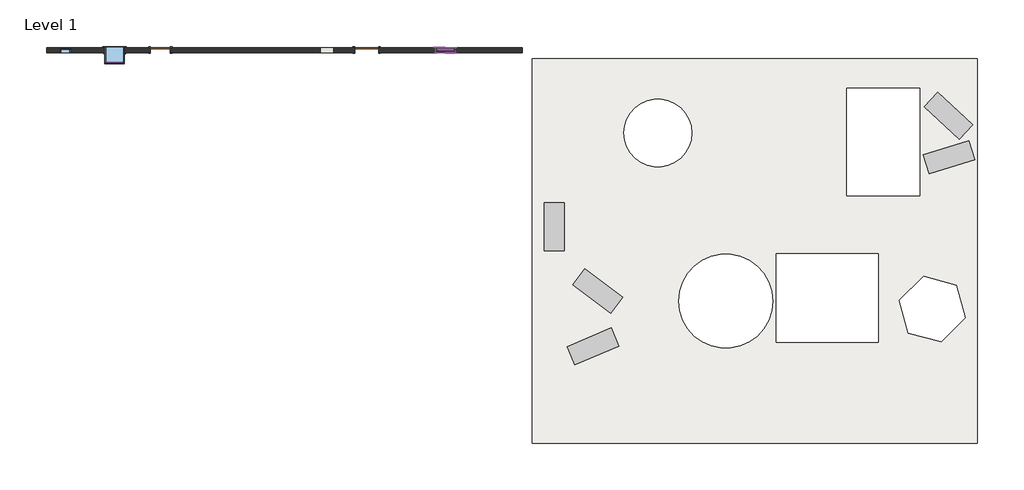
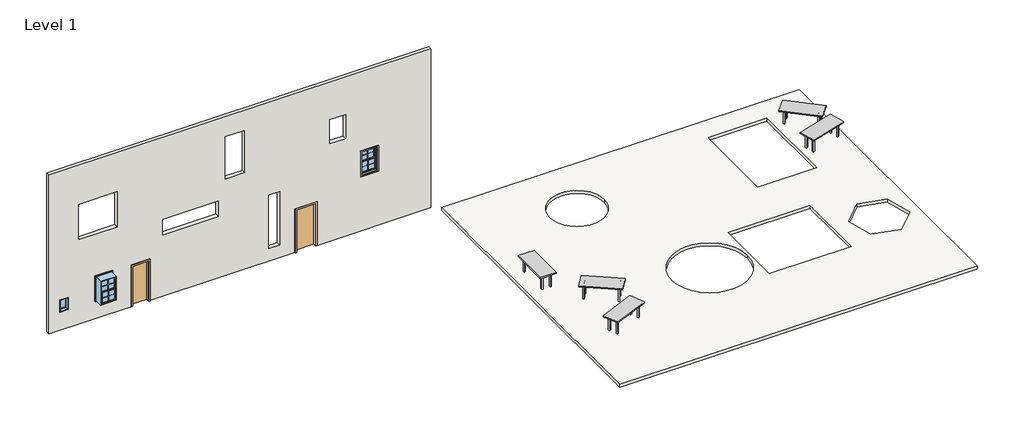
# One storey: 8 proxies, 5 furniture elements, 3 windows, 2 doors, 1 slab, 1 wall.
"""IFC4 building model written with IfcOpenShell, lengths in millimetres."""

import ifcopenshell
import ifcopenshell.guid

model = None  # the IFC model being written
_history = None  # IfcOwnerHistory: only IFC2X3 demands one
_inside = {}  # id of a spatial element -> (the spatial element, [elements in it])
_under = {}  # id of a project, library or spatial element -> (it, [spatial elements below it])
_declared = {}  # id of a project -> (the project, [libraries it declares])
_typed = {}  # id of a type object -> (the type object, [elements of that type])
_made_of = {}  # id of a material, layer set ... -> (it, [elements and type objects made of it])


def new_model(schema):
    """Start an empty IFC model of exactly this schema.

    Asked for "IFC4X3", IfcOpenShell would pick the latest addendum, in which some entities
    have other attributes; the version numbers below select the first issue.
    IFC2X3 requires an IfcOwnerHistory on every rooted entity: one is made here for all.
    """
    global model, _history
    if schema == "IFC4X3":
        model = ifcopenshell.file(schema_version=(4, 3, 0, 0))
    else:
        model = ifcopenshell.file(schema=schema)
    _inside.clear()
    _under.clear()
    _declared.clear()
    _typed.clear()
    _made_of.clear()
    _history = None
    if model.schema == "IFC2X3":
        org = make("IfcOrganization", Name="unknown")
        user = make(
            "IfcPersonAndOrganization",
            ThePerson=make("IfcPerson", FamilyName="unknown"),
            TheOrganization=org,
        )
        app = make(
            "IfcApplication",
            ApplicationDeveloper=org,
            Version="unknown",
            ApplicationFullName="unknown",
            ApplicationIdentifier="unknown",
        )
        _history = make(
            "IfcOwnerHistory",
            OwningUser=user,
            OwningApplication=app,
            ChangeAction="ADDED",
            CreationDate=0,
        )
    return model


def make(cls, **values):
    """One entity of the class cls with the attributes given. An attribute that is None is left unset."""
    return model.create_entity(
        cls, **{name: value for name, value in values.items() if value is not None}
    )


def rooted(cls, **values):
    """An entity with a GlobalId (a new one), such as an element, a storey or a relation."""
    return make(cls, GlobalId=ifcopenshell.guid.new(), OwnerHistory=_history, **values)


def si_unit(unit_type, name, prefix=None):
    """IfcSIUnit, for example si_unit("LENGTHUNIT", "METRE", prefix="MILLI")."""
    return make("IfcSIUnit", UnitType=unit_type, Prefix=prefix, Name=name)


def assignment(units):
    """IfcUnitAssignment: the units of a project."""
    return None if units is None else make("IfcUnitAssignment", Units=units)


def point(xyz):
    """IfcCartesianPoint."""
    return None if xyz is None else make("IfcCartesianPoint", Coordinates=xyz)


def direction(xyz):
    """IfcDirection."""
    return None if xyz is None else make("IfcDirection", DirectionRatios=xyz)


def frame(location, z_axis=None, x_axis=None):
    """IfcAxis2Placement3D, a coordinate frame: its origin and axes. An axis left out is left unset."""
    return make(
        "IfcAxis2Placement3D",
        Location=point(location),
        Axis=direction(z_axis),
        RefDirection=direction(x_axis),
    )


def frame_2d(location, x_axis=None):
    """IfcAxis2Placement2D, a coordinate frame in the plane: its origin and x axis."""
    return make(
        "IfcAxis2Placement2D", Location=point(location), RefDirection=direction(x_axis)
    )


def origin():
    """The frame at (0, 0, 0) with its axes left unset."""
    return frame((0.0, 0.0, 0.0))


def origin_with_axes():
    """The frame at (0, 0, 0) with the z axis (0, 0, 1) and the x axis (1, 0, 0) written out."""
    return frame((0.0, 0.0, 0.0), z_axis=(0.0, 0.0, 1.0), x_axis=(1.0, 0.0, 0.0))


def place(relative_to, where):
    """IfcLocalPlacement: puts the frame where relative to a parent placement (None: the world)."""
    return make(
        "IfcLocalPlacement", PlacementRelTo=relative_to, RelativePlacement=where
    )


def context(
    kind, dimensions, precision=None, world=None, true_north=None, identifier=None
):
    """IfcGeometricRepresentationContext, for example the 3D "Model" context."""
    return make(
        "IfcGeometricRepresentationContext",
        ContextIdentifier=identifier,
        ContextType=kind,
        CoordinateSpaceDimension=dimensions,
        Precision=precision,
        WorldCoordinateSystem=world,
        TrueNorth=true_north,
    )


def project(units=None, contexts=None):
    """IfcProject with its units and contexts."""
    return rooted(
        "IfcProject",
        Name="project",
        RepresentationContexts=contexts,
        UnitsInContext=assignment(units),
    )


def spatial(cls, under=None, at=None, **own):
    """A site, building, storey or space (cls), placed at a placement, below another one or the project."""
    s = rooted(cls, ObjectPlacement=at, **own)
    if under is not None:
        _under.setdefault(under.id(), (under, []))[1].append(s)
    return s


def polyline(points):
    """IfcPolyline through the points."""
    return make("IfcPolyline", Points=[point(p) for p in points])


def circle_curve(where, radius):
    """IfcCircle in the frame where."""
    return make("IfcCircle", Position=where, Radius=radius)


def trimmed(basis, trim1, trim2, sense, master):
    """IfcTrimmedCurve: the piece of a basis curve between two trims."""
    return make(
        "IfcTrimmedCurve",
        BasisCurve=basis,
        Trim1=trim1,
        Trim2=trim2,
        SenseAgreement=sense,
        MasterRepresentation=master,
    )


def segment(curve, same_sense, transition):
    """IfcCompositeCurveSegment."""
    return make(
        "IfcCompositeCurveSegment",
        Transition=transition,
        SameSense=same_sense,
        ParentCurve=curve,
    )


def composite_curve(segments, self_intersect=None):
    """IfcCompositeCurve: segments joined end to end."""
    return make("IfcCompositeCurve", Segments=segments, SelfIntersect=self_intersect)


def outline(outer, holes=None, kind="AREA"):
    """IfcArbitraryClosedProfileDef: a profile drawn as a closed curve; with holes, ...WithVoids."""
    if holes is None:
        return make("IfcArbitraryClosedProfileDef", ProfileType=kind, OuterCurve=outer)
    return make(
        "IfcArbitraryProfileDefWithVoids",
        ProfileType=kind,
        OuterCurve=outer,
        InnerCurves=holes,
    )


def extrude(swept, where, along, depth):
    """IfcExtrudedAreaSolid: the profile swept, set in the frame where, extruded along a direction by depth."""
    return make(
        "IfcExtrudedAreaSolid",
        SweptArea=swept,
        Position=where,
        ExtrudedDirection=direction(along),
        Depth=depth,
    )


def shape(context_of_items, identifier, shape_type, items):
    """IfcShapeRepresentation: the items that make up one representation, for example the "Body"."""
    return make(
        "IfcShapeRepresentation",
        ContextOfItems=context_of_items,
        RepresentationIdentifier=identifier,
        RepresentationType=shape_type,
        Items=items,
    )


def source(mapping_origin, context_of_items, identifier, shape_type, items):
    """IfcRepresentationMap: a shape defined once, which mapped items show again and again."""
    return make(
        "IfcRepresentationMap",
        MappingOrigin=mapping_origin,
        MappedRepresentation=shape(context_of_items, identifier, shape_type, items),
    )


def transform(
    local_origin,
    x_axis=None,
    y_axis=None,
    z_axis=None,
    scale=None,
    scale2=None,
    scale3=None,
    uniform=True,
):
    """IfcCartesianTransformationOperator3D, or its non-uniform kind. x_axis, y_axis, z_axis: its Axis1, 2, 3."""
    if uniform:
        return make(
            "IfcCartesianTransformationOperator3D",
            Axis1=direction(x_axis),
            Axis2=direction(y_axis),
            LocalOrigin=point(local_origin),
            Scale=scale,
            Axis3=direction(z_axis),
        )
    return make(
        "IfcCartesianTransformationOperator3DnonUniform",
        Axis1=direction(x_axis),
        Axis2=direction(y_axis),
        LocalOrigin=point(local_origin),
        Scale=scale,
        Axis3=direction(z_axis),
        Scale2=scale2,
        Scale3=scale3,
    )


def mapped(mapping_source, mapping_target):
    """IfcMappedItem: shows the shape of a source again, moved by a transform."""
    return make(
        "IfcMappedItem", MappingSource=mapping_source, MappingTarget=mapping_target
    )


def made_of(thing, what):
    """Note that an element or type object is made of a material, layer set ...; save() writes the relation."""
    if what is not None:
        _made_of.setdefault(what.id(), (what, []))[1].append(thing)
    return thing


def element(
    cls,
    number,
    at=None,
    inside=None,
    cuts=None,
    type_object=None,
    material=None,
    context=None,
    identifier="Body",
    shape_type=None,
    held_by="IfcProductDefinitionShape",
    body=None,
    shapes=None,
    **own,
):
    """One element of the class cls, such as IfcWall. Its Tag is "e" and its number.

    at: its placement. inside: the storey or other place that contains it. cuts: it is an
    opening in that element (IfcRelVoidsElement). A single representation is given by context,
    identifier, shape_type and body (its items); several are given by shapes. held_by: the class
    of the entity that holds the representations. save() writes the other relations.
    """
    e = rooted(cls, Tag="e%d" % number, ObjectPlacement=at, **own)
    if body is not None:
        shapes = [shape(context, identifier, shape_type, body)]
    if shapes is not None:
        e.Representation = make(held_by, Representations=shapes)
    if inside is not None:
        _inside.setdefault(inside.id(), (inside, []))[1].append(e)
    if cuts is not None:
        rooted(
            "IfcRelVoidsElement", RelatingBuildingElement=cuts, RelatedOpeningElement=e
        )
    if type_object is not None:
        _typed.setdefault(type_object.id(), (type_object, []))[1].append(e)
    return made_of(e, material)


def aggregate(whole, parts):
    """IfcRelAggregates: a whole, such as a stair, and the parts it consists of."""
    return rooted("IfcRelAggregates", RelatingObject=whole, RelatedObjects=parts)


def save(model, path):
    """Write the relations noted so far, then the file.

    IfcRelAggregates (storeys below a building ...), IfcRelContainedInSpatialStructure (elements
    in a storey), IfcRelDefinesByType, IfcRelAssociatesMaterial and IfcRelDeclares: one each for
    every whole, place, type object, material and project.
    """
    for whole, parts in _under.values():
        aggregate(whole, parts)
    for where, things in _inside.values():
        rooted(
            "IfcRelContainedInSpatialStructure",
            RelatedElements=things,
            RelatingStructure=where,
        )
    for kind, things in _typed.values():
        rooted("IfcRelDefinesByType", RelatedObjects=things, RelatingType=kind)
    for what, things in _made_of.values():
        rooted("IfcRelAssociatesMaterial", RelatedObjects=things, RelatingMaterial=what)
    for by, libraries in _declared.values():
        rooted("IfcRelDeclares", RelatingContext=by, RelatedDefinitions=libraries)
    model.write(path)


def m_muntin_pattern_2x2_m_muntin_pattern_2x2_aaec3afb(model_context):
    return source(origin(), model_context, "Body", "SweptSolid", [
        extrude(outline(polyline([(257.1375, -6.35), (257.1375, -298.8), (244.4375, -298.8), (244.4375, -6.35), (0.0, -6.35), (0.0, 6.35), (244.4375, 6.35), (244.4375, 298.8), (257.1375, 298.8), (257.1375, 6.35), (501.575, 6.35), (501.575, -6.35), (257.1375, -6.35)])), frame((0.0, 9.525, 0.0), z_axis=(0.0, 1.0, 0.0), x_axis=(0.0, 0.0, 1.0)), (0.0, 0.0, 1.0), 12.7),
        extrude(outline(polyline([(257.1375, -6.35), (257.1375, -298.8), (244.4375, -298.8), (244.4375, -6.35), (0.0, -6.35), (0.0, 6.35), (244.4375, 6.35), (244.4375, 298.8), (257.1375, 298.8), (257.1375, 6.35), (501.575, 6.35), (501.575, -6.35), (257.1375, -6.35)])), frame((0.0, -22.225, 0.0), z_axis=(0.0, 1.0, 0.0), x_axis=(0.0, 0.0, 1.0)), (0.0, 0.0, 1.0), 12.7),
    ])


def m_trim_window_exterior_flat_with_sill_e7ff6350(model_context):
    return source(origin(), model_context, "Body", "SweptSolid", [
        extrude(outline(polyline([(435.0, -1220.4323709), (435.0, -1280.4323709), (-435.0, -1280.4323709), (-435.0, -1220.4323709), (435.0, -1220.4323709)])), origin_with_axes(), (0.0, 0.0, 1.0), 19.05),
        extrude(outline(polyline([(-1230.0, 38.1), (-1202.4580645, 38.1), (-1200.0, 19.05), (-1200.0, 0.0), (-1220.4323709, 0.0), (-1220.4323709, 19.05), (-1230.0, 19.05), (-1230.0, 38.1)])), frame((-447.7, 0.0, 0.0), z_axis=(1.0, 0.0, 0.0), x_axis=(0.0, 1.0, 0.0)), (0.0, 0.0, 1.0), 895.4),
        extrude(outline(polyline([(-435.0, 60.0), (435.0, 60.0), (435.0, -1200.0), (375.0, -1200.0), (375.0, 0.0), (-375.0, 0.0), (-375.0, -1200.0), (-435.0, -1200.0), (-435.0, 60.0)])), origin_with_axes(), (0.0, 0.0, 1.0), 19.05),
    ])


def m_trim_window_interior_flat_picture_frame_31bd2320(model_context):
    return source(origin(), model_context, "Body", "SweptSolid", [
        extrude(outline(polyline([(422.3, 47.3), (422.3, -1247.3), (-422.3, -1247.3), (-422.3, 47.3), (422.3, 47.3)]), holes=[polyline([(362.3, -12.7), (-362.3, -12.7), (-362.3, -1187.3), (362.3, -1187.3), (362.3, -12.7)])]), origin_with_axes(), (0.0, 0.0, 1.0), 30.0),
    ])


def m_single_flush_0762_x_2032mm_0c256fab(model_context):
    return source(origin(), model_context, "Body", "SweptSolid", [
        extrude(outline(polyline([(2108.0, -457.0), (0.0, -457.0), (0.0, -381.0), (2032.0, -381.0), (2032.0, 381.0), (0.0, 381.0), (0.0, 457.0), (2108.0, 457.0), (2108.0, -457.0)])), frame((0.0, 100.0, 0.0), z_axis=(0.0, 1.0, 0.0), x_axis=(0.0, 0.0, 1.0)), (0.0, 0.0, 1.0), 25.0),
        extrude(outline(polyline([(2108.0, 457.0), (2108.0, -457.0), (0.0, -457.0), (0.0, -381.0), (2032.0, -381.0), (2032.0, 381.0), (0.0, 381.0), (0.0, 457.0), (2108.0, 457.0)])), frame((0.0, -125.0, 0.0), z_axis=(0.0, 1.0, 0.0), x_axis=(0.0, 0.0, 1.0)), (0.0, 0.0, 1.0), 25.0),
        extrude(outline(polyline([(381.0, 49.0), (-381.0, 49.0), (-381.0, 100.0), (381.0, 100.0), (381.0, 49.0)])), origin_with_axes(), (0.0, 0.0, 1.0), 2032.0),
    ])


def m_single_flush_0915_x_2134mm_727434cd(model_context):
    return source(origin(), model_context, "Body", "SweptSolid", [
        extrude(outline(polyline([(2210.0, -533.5), (0.0, -533.5), (0.0, -457.5), (2134.0, -457.5), (2134.0, 457.5), (0.0, 457.5), (0.0, 533.5), (2210.0, 533.5), (2210.0, -533.5)])), frame((0.0, -125.0, 0.0), z_axis=(0.0, 1.0, 0.0), x_axis=(0.0, 0.0, 1.0)), (0.0, 0.0, 1.0), 25.0),
        extrude(outline(polyline([(2210.0, 533.5), (2210.0, -533.5), (0.0, -533.5), (0.0, -457.5), (2134.0, -457.5), (2134.0, 457.5), (0.0, 457.5), (0.0, 533.5), (2210.0, 533.5)])), frame((0.0, 100.0, 0.0), z_axis=(0.0, 1.0, 0.0), x_axis=(0.0, 0.0, 1.0)), (0.0, 0.0, 1.0), 25.0),
        extrude(outline(polyline([(457.5, -49.0), (457.5, -100.0), (-457.5, -100.0), (-457.5, -49.0), (457.5, -49.0)])), origin_with_axes(), (0.0, 0.0, 1.0), 2134.0),
    ])


def m_table_rectangular_1830_x_0762mm_a0b3b7a0(model_context):
    return source(origin(), model_context, "Body", "SweptSolid", [
        extrude(outline(polyline([(699.1, 190.5), (699.1, 165.1), (-699.1, 165.1), (-699.1, 190.5), (699.1, 190.5)])), frame((0.0, 0.0, 609.6), z_axis=(0.0, 0.0, 1.0), x_axis=(1.0, 0.0, 0.0)), (0.0, 0.0, 1.0), 101.6),
        extrude(outline(polyline([(699.1, -190.5), (-699.1, -190.5), (-699.1, -165.1), (699.1, -165.1), (699.1, -190.5)])), frame((0.0, 0.0, 609.6), z_axis=(0.0, 0.0, 1.0), x_axis=(1.0, 0.0, 0.0)), (0.0, 0.0, 1.0), 101.6),
        extrude(outline(polyline([(-711.8, -165.1), (-737.2, -165.1), (-737.2, 165.1), (-711.8, 165.1), (-711.8, -165.1)])), frame((0.0, 0.0, 609.6), z_axis=(0.0, 0.0, 1.0), x_axis=(1.0, 0.0, 0.0)), (0.0, 0.0, 1.0), 101.6),
        extrude(outline(polyline([(711.8, -165.1), (711.8, 165.1), (737.2, 165.1), (737.2, -165.1), (711.8, -165.1)])), frame((0.0, 0.0, 609.6), z_axis=(0.0, 0.0, 1.0), x_axis=(1.0, 0.0, 0.0)), (0.0, 0.0, 1.0), 101.6),
        extrude(outline(polyline([(915.0, 381.0), (915.0, -381.0), (-915.0, -381.0), (-915.0, 381.0), (915.0, 381.0)])), frame((0.0, 0.0, 711.2), z_axis=(0.0, 0.0, 1.0), x_axis=(1.0, 0.0, 0.0)), (0.0, 0.0, 1.0), 50.8),
        extrude(outline(polyline([(-699.1, 228.6), (-699.1, 165.1), (-762.6, 165.1), (-762.6, 228.6), (-699.1, 228.6)])), origin_with_axes(), (0.0, 0.0, 1.0), 711.2),
        extrude(outline(polyline([(699.1, 228.6), (762.6, 228.6), (762.6, 165.1), (699.1, 165.1), (699.1, 228.6)])), origin_with_axes(), (0.0, 0.0, 1.0), 711.2),
        extrude(outline(polyline([(-699.1, -228.6), (-762.6, -228.6), (-762.6, -165.1), (-699.1, -165.1), (-699.1, -228.6)])), origin_with_axes(), (0.0, 0.0, 1.0), 711.2),
        extrude(outline(polyline([(699.1, -228.6), (699.1, -165.1), (762.6, -165.1), (762.6, -228.6), (699.1, -228.6)])), origin_with_axes(), (0.0, 0.0, 1.0), 711.2),
    ])


def m_table_rectangular_1830_x_0762mm_ec068ed4(model_context):
    return source(origin(), model_context, "Body", "SweptSolid", [
        extrude(outline(polyline([(699.1, -190.5), (-699.1, -190.5), (-699.1, -165.1), (699.1, -165.1), (699.1, -190.5)])), frame((0.0, 0.0, 609.6), z_axis=(0.0, 0.0, 1.0), x_axis=(1.0, 0.0, 0.0)), (0.0, 0.0, 1.0), 101.6),
        extrude(outline(polyline([(699.1, 190.5), (699.1, 165.1), (-699.1, 165.1), (-699.1, 190.5), (699.1, 190.5)])), frame((0.0, 0.0, 609.6), z_axis=(0.0, 0.0, 1.0), x_axis=(1.0, 0.0, 0.0)), (0.0, 0.0, 1.0), 101.6),
        extrude(outline(polyline([(-711.8, 165.1), (-711.8, -165.1), (-737.2, -165.1), (-737.2, 165.1), (-711.8, 165.1)])), frame((0.0, 0.0, 609.6), z_axis=(0.0, 0.0, 1.0), x_axis=(1.0, 0.0, 0.0)), (0.0, 0.0, 1.0), 101.6),
        extrude(outline(polyline([(711.8, 165.1), (737.2, 165.1), (737.2, -165.1), (711.8, -165.1), (711.8, 165.1)])), frame((0.0, 0.0, 609.6), z_axis=(0.0, 0.0, 1.0), x_axis=(1.0, 0.0, 0.0)), (0.0, 0.0, 1.0), 101.6),
        extrude(outline(polyline([(915.0, -381.0), (-915.0, -381.0), (-915.0, 381.0), (915.0, 381.0), (915.0, -381.0)])), frame((0.0, 0.0, 711.2), z_axis=(0.0, 0.0, 1.0), x_axis=(1.0, 0.0, 0.0)), (0.0, 0.0, 1.0), 50.8),
        extrude(outline(polyline([(-699.1, -228.6), (-762.6, -228.6), (-762.6, -165.1), (-699.1, -165.1), (-699.1, -228.6)])), origin_with_axes(), (0.0, 0.0, 1.0), 711.2),
        extrude(outline(polyline([(699.1, -228.6), (699.1, -165.1), (762.6, -165.1), (762.6, -228.6), (699.1, -228.6)])), origin_with_axes(), (0.0, 0.0, 1.0), 711.2),
        extrude(outline(polyline([(-699.1, 228.6), (-699.1, 165.1), (-762.6, 165.1), (-762.6, 228.6), (-699.1, 228.6)])), origin_with_axes(), (0.0, 0.0, 1.0), 711.2),
        extrude(outline(polyline([(699.1, 228.6), (762.6, 228.6), (762.6, 165.1), (699.1, 165.1), (699.1, 228.6)])), origin_with_axes(), (0.0, 0.0, 1.0), 711.2),
    ])


def m_fixed_0406_x_0610mm_8205b201(model_context):
    return source(origin(), model_context, "Body", "SweptSolid", [
        extrude(outline(polyline([(-140.0, 78.0), (140.0, 78.0), (140.0, 66.0), (-140.0, 66.0), (-140.0, 78.0)])), frame((0.0, 0.0, 978.0), z_axis=(0.0, 0.0, 1.0), x_axis=(1.0, 0.0, 0.0)), (0.0, 0.0, 1.0), 484.0),
        extrude(outline(polyline([(1506.0, -184.0), (934.0, -184.0), (934.0, 184.0), (1506.0, 184.0), (1506.0, -184.0)]), holes=[polyline([(1462.0, -140.0), (1462.0, 140.0), (978.0, 140.0), (978.0, -140.0), (1462.0, -140.0)])]), frame((0.0, 50.0, 0.0), z_axis=(0.0, 1.0, 0.0), x_axis=(0.0, 0.0, 1.0)), (0.0, 0.0, 1.0), 44.0),
        extrude(outline(polyline([(1525.0, -203.0), (915.0, -203.0), (915.0, 203.0), (1525.0, 203.0), (1525.0, -203.0)]), holes=[polyline([(1506.0, -184.0), (1506.0, 184.0), (934.0, 184.0), (934.0, -184.0), (1506.0, -184.0)])]), frame((0.0, 50.0, 0.0), z_axis=(0.0, 1.0, 0.0), x_axis=(0.0, 0.0, 1.0)), (0.0, 0.0, 1.0), 63.0),
        extrude(outline(polyline([(1525.0, -203.0), (915.0, -203.0), (915.0, 203.0), (1525.0, 203.0), (1525.0, -203.0)]), holes=[polyline([(1493.0, -171.0), (1493.0, 171.0), (947.0, 171.0), (947.0, -171.0), (1493.0, -171.0)])]), frame((0.0, -87.0, 0.0), z_axis=(0.0, 1.0, 0.0), x_axis=(0.0, 0.0, 1.0)), (0.0, 0.0, 1.0), 137.0),
    ])


def m_window_double_hung_750_x_1200mm_e21ea802(model_context):
    return source(origin(), model_context, "Body", "SweptSolid", [
        extrude(outline(polyline([(298.8, -469.85), (298.8, -476.2), (-298.8, -476.2), (-298.8, -469.85), (298.8, -469.85)])), frame((0.0, 0.0, 990.6), z_axis=(0.0, 0.0, 1.0), x_axis=(1.0, 0.0, 0.0)), (0.0, 0.0, 1.0), 501.575),
        extrude(outline(polyline([(-298.8, -482.55), (298.8, -482.55), (298.8, -488.9), (-298.8, -488.9), (-298.8, -482.55)])), frame((0.0, 0.0, 990.6), z_axis=(0.0, 0.0, 1.0), x_axis=(1.0, 0.0, 0.0)), (0.0, 0.0, 1.0), 501.575),
        extrude(outline(polyline([(298.8, -425.4), (298.8, -431.75), (-298.8, -431.75), (-298.8, -425.4), (298.8, -425.4)])), frame((0.0, 0.0, 1536.625), z_axis=(0.0, 0.0, 1.0), x_axis=(1.0, 0.0, 0.0)), (0.0, 0.0, 1.0), 501.575),
        extrude(outline(polyline([(-298.8, -438.1), (298.8, -438.1), (298.8, -444.45), (-298.8, -444.45), (-298.8, -438.1)])), frame((0.0, 0.0, 1536.625), z_axis=(0.0, 0.0, 1.0), x_axis=(1.0, 0.0, 0.0)), (0.0, 0.0, 1.0), 501.575),
        extrude(outline(polyline([(1536.625, -343.25), (946.15, -343.25), (946.15, 343.25), (1536.625, 343.25), (1536.625, -343.25)]), holes=[polyline([(1492.175, 298.8), (990.6, 298.8), (990.6, -298.8), (1492.175, -298.8), (1492.175, 298.8)])]), frame((0.0, -501.6, 0.0), z_axis=(0.0, 1.0, 0.0), x_axis=(0.0, 0.0, 1.0)), (0.0, 0.0, 1.0), 44.45),
        extrude(outline(polyline([(2082.65, -343.25), (1492.175, -343.25), (1492.175, 343.25), (2082.65, 343.25), (2082.65, -343.25)]), holes=[polyline([(2038.2, 298.8), (1536.625, 298.8), (1536.625, -298.8), (2038.2, -298.8), (2038.2, 298.8)])]), frame((0.0, -457.15, 0.0), z_axis=(0.0, 1.0, 0.0), x_axis=(0.0, 0.0, 1.0)), (0.0, 0.0, 1.0), 44.45),
        extrude(outline(polyline([(2114.4, -375.0), (914.4, -375.0), (914.4, 375.0), (2114.4, 375.0), (2114.4, -375.0)]), holes=[polyline([(2082.65, 343.25), (946.15, 343.25), (946.15, -343.25), (2082.65, -343.25), (2082.65, 343.25)])]), frame((0.0, -514.3, 0.0), z_axis=(0.0, 1.0, 0.0), x_axis=(0.0, 0.0, 1.0)), (0.0, 0.0, 1.0), 633.35),
    ])


def m_window_double_hung_750_x_1200mm_41070976(model_context):
    return source(origin(), model_context, "Body", "SweptSolid", [
        extrude(outline(polyline([(298.8, 30.15), (298.8, 23.8), (-298.8, 23.8), (-298.8, 30.15), (298.8, 30.15)])), frame((0.0, 0.0, 990.6), z_axis=(0.0, 0.0, 1.0), x_axis=(1.0, 0.0, 0.0)), (0.0, 0.0, 1.0), 501.575),
        extrude(outline(polyline([(-298.8, 17.45), (298.8, 17.45), (298.8, 11.1), (-298.8, 11.1), (-298.8, 17.45)])), frame((0.0, 0.0, 990.6), z_axis=(0.0, 0.0, 1.0), x_axis=(1.0, 0.0, 0.0)), (0.0, 0.0, 1.0), 501.575),
        extrude(outline(polyline([(298.8, 74.6), (298.8, 68.25), (-298.8, 68.25), (-298.8, 74.6), (298.8, 74.6)])), frame((0.0, 0.0, 1536.625), z_axis=(0.0, 0.0, 1.0), x_axis=(1.0, 0.0, 0.0)), (0.0, 0.0, 1.0), 501.575),
        extrude(outline(polyline([(-298.8, 61.9), (298.8, 61.9), (298.8, 55.55), (-298.8, 55.55), (-298.8, 61.9)])), frame((0.0, 0.0, 1536.625), z_axis=(0.0, 0.0, 1.0), x_axis=(1.0, 0.0, 0.0)), (0.0, 0.0, 1.0), 501.575),
        extrude(outline(polyline([(1536.625, -343.25), (946.15, -343.25), (946.15, 343.25), (1536.625, 343.25), (1536.625, -343.25)]), holes=[polyline([(1492.175, 298.8), (990.6, 298.8), (990.6, -298.8), (1492.175, -298.8), (1492.175, 298.8)])]), frame((0.0, -1.6, 0.0), z_axis=(0.0, 1.0, 0.0), x_axis=(0.0, 0.0, 1.0)), (0.0, 0.0, 1.0), 44.45),
        extrude(outline(polyline([(2082.65, -343.25), (1492.175, -343.25), (1492.175, 343.25), (2082.65, 343.25), (2082.65, -343.25)]), holes=[polyline([(2038.2, 298.8), (1536.625, 298.8), (1536.625, -298.8), (2038.2, -298.8), (2038.2, 298.8)])]), frame((0.0, 42.85, 0.0), z_axis=(0.0, 1.0, 0.0), x_axis=(0.0, 0.0, 1.0)), (0.0, 0.0, 1.0), 44.45),
        extrude(outline(polyline([(2114.4, -375.0), (914.4, -375.0), (914.4, 375.0), (2114.4, 375.0), (2114.4, -375.0)]), holes=[polyline([(2082.65, 343.25), (946.15, 343.25), (946.15, -343.25), (2082.65, -343.25), (2082.65, 343.25)])]), frame((0.0, -14.3, 0.0), z_axis=(0.0, 1.0, 0.0), x_axis=(0.0, 0.0, 1.0)), (0.0, 0.0, 1.0), 133.35),
        extrude(outline(polyline([(2114.4, 375.0), (2114.4, -375.0), (914.4, -375.0), (914.4, 375.0), (2114.4, 375.0)]), holes=[polyline([(2095.35, 355.95), (933.45, 355.95), (933.45, -355.95), (2095.35, -355.95), (2095.35, 355.95)])]), frame((0.0, -100.0, 0.0), z_axis=(0.0, 1.0, 0.0), x_axis=(0.0, 0.0, 1.0)), (0.0, 0.0, 1.0), 85.7),
    ])


model = new_model("IFC4")

# Units and contexts
model_context = context("Model", 3, world=origin())
ifc_project = project(units=[si_unit("LENGTHUNIT", "METRE", prefix="MILLI")], contexts=[model_context])

# Site, building, storey
site = spatial("IfcSite", under=ifc_project)
building = spatial("IfcBuilding", under=site)
storey = spatial("IfcBuildingStorey", under=building, Name="Level 1", Elevation=0.0)

# Proxies
placement = place(None, origin())
m_muntin_pattern_2x2_m_muntin_pattern_2x2_shape = m_muntin_pattern_2x2_m_muntin_pattern_2x2_aaec3afb(model_context)
element("IfcBuildingElementProxy", 1, Name="M_Muntin Pattern_2x2 : M_Muntin Pattern_2x2", ObjectType="M_Muntin Pattern_2x2 : M_Muntin Pattern_2x2", at=placement, inside=storey, context=model_context, shape_type="MappedRepresentation", body=[
    mapped(m_muntin_pattern_2x2_m_muntin_pattern_2x2_shape, transform((-13755.2543844, 2099.5505832, 3404.9440493), x_axis=(1.0, 0.0, 0.0), y_axis=(0.0, 1.0, 0.0), z_axis=(0.0, 0.0, 1.0))),
])
element("IfcBuildingElementProxy", 2, Name="M_Muntin Pattern_2x2 : M_Muntin Pattern_2x2", ObjectType="M_Muntin Pattern_2x2 : M_Muntin Pattern_2x2", at=placement, inside=storey, context=model_context, shape_type="MappedRepresentation", body=[
    mapped(m_muntin_pattern_2x2_m_muntin_pattern_2x2_shape, transform((-13755.2543844, 2055.1005832, 2858.9190493), x_axis=(1.0, 0.0, 0.0), y_axis=(0.0, 1.0, 0.0), z_axis=(0.0, 0.0, 1.0))),
])
element("IfcBuildingElementProxy", 3, Name="M_Muntin Pattern_2x2 : M_Muntin Pattern_2x2", ObjectType="M_Muntin Pattern_2x2 : M_Muntin Pattern_2x2", at=placement, inside=storey, context=model_context, shape_type="MappedRepresentation", body=[
    mapped(m_muntin_pattern_2x2_m_muntin_pattern_2x2_shape, transform((-26415.5284847, 1599.5505832, 1536.625), x_axis=(1.0, 0.0, 0.0), y_axis=(0.0, 1.0, 0.0), z_axis=(0.0, 0.0, 1.0))),
])
element("IfcBuildingElementProxy", 4, Name="M_Muntin Pattern_2x2 : M_Muntin Pattern_2x2", ObjectType="M_Muntin Pattern_2x2 : M_Muntin Pattern_2x2", at=placement, inside=storey, context=model_context, shape_type="MappedRepresentation", body=[
    mapped(m_muntin_pattern_2x2_m_muntin_pattern_2x2_shape, transform((-26415.5284847, 1555.1005832, 990.6), x_axis=(1.0, 0.0, 0.0), y_axis=(0.0, 1.0, 0.0), z_axis=(0.0, 0.0, 1.0))),
])
m_trim_window_exterior_flat_with_sill_shape = m_trim_window_exterior_flat_with_sill_e7ff6350(model_context)
element("IfcBuildingElementProxy", 5, Name="M_Trim-Window-Exterior-Flat : with Sill", ObjectType="M_Trim-Window-Exterior-Flat : with Sill", at=placement, inside=storey, context=model_context, shape_type="MappedRepresentation", body=[
    mapped(m_trim_window_exterior_flat_with_sill_shape, transform((-13755.2543844, 2134.4755832, 3982.7190493), x_axis=(-1.0, 0.0, 0.0), y_axis=(0.0, 0.0, 1.0), z_axis=(0.0, 1.0, 0.0))),
])
element("IfcBuildingElementProxy", 6, Name="M_Trim-Window-Exterior-Flat : with Sill", ObjectType="M_Trim-Window-Exterior-Flat : with Sill", at=placement, inside=storey, context=model_context, shape_type="MappedRepresentation", body=[
    mapped(m_trim_window_exterior_flat_with_sill_shape, transform((-26415.5284847, 2134.4755832, 2114.4), x_axis=(-1.0, 0.0, 0.0), y_axis=(0.0, 0.0, 1.0), z_axis=(0.0, 1.0, 0.0))),
])
m_trim_window_interior_flat_picture_frame_shape = m_trim_window_interior_flat_picture_frame_31bd2320(model_context)
element("IfcBuildingElementProxy", 7, Name="M_Trim-Window-Interior-Flat : Picture Frame", ObjectType="M_Trim-Window-Interior-Flat : Picture Frame", at=placement, inside=storey, context=model_context, shape_type="MappedRepresentation", body=[
    mapped(m_trim_window_interior_flat_picture_frame_shape, transform((-13755.2543844, 1934.4755832, 3982.7190493), x_axis=(1.0, 0.0, 0.0), y_axis=(0.0, 0.0, 1.0), z_axis=(0.0, -1.0, 0.0))),
])
element("IfcBuildingElementProxy", 8, Name="M_Trim-Window-Interior-Flat : Picture Frame", ObjectType="M_Trim-Window-Interior-Flat : Picture Frame", at=placement, inside=storey, context=model_context, shape_type="MappedRepresentation", body=[
    mapped(m_trim_window_interior_flat_picture_frame_shape, transform((-26415.5284847, 1934.4755832, 2114.4), x_axis=(1.0, 0.0, 0.0), y_axis=(0.0, 0.0, 1.0), z_axis=(0.0, -1.0, 0.0))),
])

# Doors
m_single_flush_0762_x_2032mm_shape = m_single_flush_0762_x_2032mm_0c256fab(model_context)
element("IfcDoor", 9, ObjectType="M_Single-Flush : 0762 x 2032mm", at=placement, inside=storey, context=model_context, shape_type="MappedRepresentation", body=[
    mapped(m_single_flush_0762_x_2032mm_shape, transform((-24659.5284847, 2034.4755832, 0.0), x_axis=(1.0, 0.0, 0.0), y_axis=(0.0, 1.0, 0.0), z_axis=(0.0, 0.0, 1.0))),
])
m_single_flush_0915_x_2134mm_shape = m_single_flush_0915_x_2134mm_727434cd(model_context)
element("IfcDoor", 10, ObjectType="M_Single-Flush : 0915 x 2134mm", at=placement, inside=storey, context=model_context, shape_type="MappedRepresentation", body=[
    mapped(m_single_flush_0915_x_2134mm_shape, transform((-16774.8897659, 2034.4755832, 0.0), x_axis=(-1.0, 0.0, 0.0), y_axis=(0.0, -1.0, 0.0), z_axis=(0.0, 0.0, 1.0))),
])

# Furniture
m_table_rectangular_1830_x_0762mm_shape = m_table_rectangular_1830_x_0762mm_a0b3b7a0(model_context)
element("IfcFurniture", 11, ObjectType="M_Table-Rectangular : 1830 x 0762mm", at=placement, inside=storey, context=model_context, shape_type="MappedRepresentation", body=[
    mapped(m_table_rectangular_1830_x_0762mm_shape, transform((-7934.3893105, -7176.9572862, 0.0), x_axis=(0.7986355100472892, -0.601815023152053, 0.0), y_axis=(0.601815023152053, 0.7986355100472892, 0.0), z_axis=(0.0, 0.0, 1.0))),
])
element("IfcFurniture", 12, ObjectType="M_Table-Rectangular : 1830 x 0762mm", at=placement, inside=storey, context=model_context, shape_type="MappedRepresentation", body=[
    mapped(m_table_rectangular_1830_x_0762mm_shape, transform((-9596.1972949, -4723.9774044, 0.0), x_axis=(0.0, 1.0, 0.0), y_axis=(-1.0, 0.0, 0.0), z_axis=(0.0, 0.0, 1.0))),
])
element("IfcFurniture", 13, ObjectType="M_Table-Rectangular : 1830 x 0762mm", at=placement, inside=storey, context=model_context, shape_type="MappedRepresentation", body=[
    mapped(m_table_rectangular_1830_x_0762mm_shape, transform((-8112.0141227, -9301.6688903, 0.0), x_axis=(0.9205048534524458, 0.39073112848926067, 0.0), y_axis=(-0.39073112848926067, 0.9205048534524458, 0.0), z_axis=(0.0, 0.0, 1.0))),
])
m_table_rectangular_1830_x_0762mm_2_shape = m_table_rectangular_1830_x_0762mm_ec068ed4(model_context)
element("IfcFurniture", 14, ObjectType="M_Table-Rectangular : 1830 x 0762mm", at=placement, inside=storey, context=model_context, shape_type="MappedRepresentation", body=[
    mapped(m_table_rectangular_1830_x_0762mm_2_shape, transform((5509.5543182, -2054.6922097, 0.0), x_axis=(-0.9563047559630324, -0.2923717047227468, 0.0), y_axis=(0.2923717047227468, -0.9563047559630324, 0.0), z_axis=(0.0, 0.0, 1.0))),
])
element("IfcFurniture", 15, ObjectType="M_Table-Rectangular : 1830 x 0762mm", at=placement, inside=storey, context=model_context, shape_type="MappedRepresentation", body=[
    mapped(m_table_rectangular_1830_x_0762mm_2_shape, transform((5492.8202713, -469.7512134, 0.0), x_axis=(-0.7313537016191695, 0.6819983600624996, 0.0), y_axis=(-0.6819983600624996, -0.7313537016191695, 0.0), z_axis=(0.0, 0.0, 1.0))),
])

# Slab
element("IfcSlab", 16, ObjectType="Generic 150mm", at=placement, inside=storey, context=model_context, shape_type="SweptSolid", body=[
    extrude(outline(polyline([(-10438.0920872, 1704.9536342), (6597.1361468, 1704.9536342), (6597.1361468, -12995.0463658), (-10438.0920872, -12995.0463658), (-10438.0920872, 1704.9536342)]), holes=[polyline([(-1096.2822975, -5745.5612839), (-1096.2822975, -9145.5612839), (2803.7177025, -9145.5612839), (2803.7177025, -5745.5612839), (-1096.2822975, -5745.5612839)]), composite_curve([segment(trimmed(circle_curve(frame_2d((-3026.5132944, -7566.8871411)), 1800.0), [point((-1226.5132944, -7566.8871411))], [point((-4826.5132944, -7566.8871411))], True, "CARTESIAN"), True, "CONTINUOUS"), segment(trimmed(circle_curve(frame_2d((-3026.5132944, -7566.8871411)), 1800.0), [point((-4826.5132944, -7566.8871411))], [point((-1226.5132944, -7566.8871411))], True, "CARTESIAN"), True, "CONTINUOUS")], self_intersect=False), polyline([(3950.2905395, -8793.2666419), (5205.9941136, -9129.7314005), (6125.2329292, -8210.492585), (5788.7681706, -6954.7890108), (4533.0645964, -6618.3242522), (3613.8257808, -7537.5630677), (3950.2905395, -8793.2666419)]), polyline([(4397.1361468, 574.3329665), (1597.1361468, 574.3329665), (1597.1361468, -3525.6670335), (4397.1361468, -3525.6670335), (4397.1361468, 574.3329665)]), composite_curve([segment(trimmed(circle_curve(frame_2d((-5632.920233, -1133.8213408)), 1300.0), [point((-4332.920233, -1133.8213408))], [point((-6932.920233, -1133.8213408))], True, "CARTESIAN"), True, "CONTINUOUS"), segment(trimmed(circle_curve(frame_2d((-5632.920233, -1133.8213408)), 1300.0), [point((-6932.920233, -1133.8213408))], [point((-4332.920233, -1133.8213408))], True, "CARTESIAN"), True, "CONTINUOUS")], self_intersect=False)]), frame((0.0, 0.0, -150.0), z_axis=(0.0, 0.0, 1.0), x_axis=(1.0, 0.0, 0.0)), (0.0, 0.0, 1.0), 150.0),
])

# Wall
element("IfcWall", 17, ObjectType="Generic - 200mm", at=placement, inside=storey, context=model_context, shape_type="SweptSolid", body=[
    extrude(outline(polyline([(8000.0, -29017.3897659), (0.0, -29017.3897659), (0.0, -25040.5284847), (2032.0, -25040.5284847), (2032.0, -24278.5284847), (0.0, -24278.5284847), (0.0, -17232.3897659), (2134.0, -17232.3897659), (2134.0, -16317.3897659), (0.0, -16317.3897659), (0.0, -10817.3897659), (8000.0, -10817.3897659), (8000.0, -29017.3897659)]), holes=[polyline([(915.0, -28496.5284847), (1525.0, -28496.5284847), (1525.0, -28090.5284847), (915.0, -28090.5284847), (915.0, -28496.5284847)]), polyline([(914.4, -26790.5284847), (2114.4, -26790.5284847), (2114.4, -26040.5284847), (914.4, -26040.5284847), (914.4, -26790.5284847)]), polyline([(2782.7190493, -14130.2543844), (3982.7190493, -14130.2543844), (3982.7190493, -13380.2543844), (2782.7190493, -13380.2543844), (2782.7190493, -14130.2543844)]), polyline([(4914.4, -15639.9853759), (6114.4, -15639.9853759), (6114.4, -14889.9853759), (4914.4, -14889.9853759), (4914.4, -15639.9853759)]), polyline([(4866.0, -19702.3897659), (4866.0, -20617.3897659), (7000.0, -20617.3897659), (7000.0, -19702.3897659), (4866.0, -19702.3897659)]), polyline([(3328.9271244, -18544.8897659), (3328.9271244, -18024.3599995), (634.0, -18024.3599995), (634.0, -18544.8897659), (3328.9271244, -18544.8897659)]), polyline([(3873.453269, -23605.3752389), (3873.453269, -20944.8897659), (3100.0, -20944.8897659), (3100.0, -23605.3752389), (3873.453269, -23605.3752389)]), polyline([(6036.9886823, -27608.1535838), (6036.9886823, -25757.3810809), (4260.1064286, -25757.3810809), (4260.1064286, -27608.1535838), (6036.9886823, -27608.1535838)])]), frame((0.0, 1934.4755832, 0.0), z_axis=(0.0, 1.0, 0.0), x_axis=(0.0, 0.0, 1.0)), (0.0, 0.0, 1.0), 200.0),
])

# Windows
m_fixed_0406_x_0610mm_shape = m_fixed_0406_x_0610mm_8205b201(model_context)
element("IfcWindow", 18, ObjectType="M_Fixed : 0406 x 0610mm", at=placement, inside=storey, context=model_context, shape_type="MappedRepresentation", body=[
    mapped(m_fixed_0406_x_0610mm_shape, transform((-28293.5284847, 2021.4755832, 0.0), x_axis=(1.0, 0.0, 0.0), y_axis=(0.0, 1.0, 0.0), z_axis=(0.0, 0.0, 1.0))),
])
m_window_double_hung_750_x_1200mm_shape = m_window_double_hung_750_x_1200mm_e21ea802(model_context)
element("IfcWindow", 19, ObjectType="M_Window-Double-Hung : 750 x 1200mm", at=placement, inside=storey, context=model_context, shape_type="MappedRepresentation", body=[
    mapped(m_window_double_hung_750_x_1200mm_shape, transform((-26415.5284847, 2034.4755832, 0.0), x_axis=(1.0, 0.0, 0.0), y_axis=(0.0, 1.0, 0.0), z_axis=(0.0, 0.0, 1.0))),
])
m_window_double_hung_750_x_1200mm_2_shape = m_window_double_hung_750_x_1200mm_41070976(model_context)
element("IfcWindow", 20, ObjectType="M_Window-Double-Hung : 750 x 1200mm", at=placement, inside=storey, context=model_context, shape_type="MappedRepresentation", body=[
    mapped(m_window_double_hung_750_x_1200mm_2_shape, transform((-13755.2543844, 2034.4755832, 1868.3190493), x_axis=(1.0, 0.0, 0.0), y_axis=(0.0, 1.0, 0.0), z_axis=(0.0, 0.0, 1.0))),
])

save(model, "model.ifc")

# Revit data of these elements
# Project information
#   Project Issue Date = "Issue Date"
#   Project Status = "Project Status"
#   Client Name = "Owner"
#   Project Address = "Enter address here"
#   Project Name = "Project Name"
#   Project Number = "0001"
# Type "M_Muntin Pattern_2x2 : M_Muntin Pattern_2x2"
#   Width [instance default] = 1200 mm
#   Thickness = 12.7 mm
#   Height [instance default] = 1200 mm
#   Distance = 19.05 mm
#   Interior Material [instance default] = none
#   Exterior Material [instance default] = none
#   Default Elevation = 0
# Type "M_Trim-Window-Exterior-Flat : with Sill"
#   Trim Width = 60 mm
#   Trim Thickness_Picture Frame = 30 mm
#   Trim Thickness_with Sill = 19.05 mm
#   Sill Thickness = 30 mm
#   Opening Width [instance default] = 600 mm
#   Opening Height [instance default] = 900 mm
#   Default Elevation = 1200 mm
#   Sill = yes
#   Picture Frame = no
#   Trim Material [instance default] = none
# Type "M_Trim-Window-Interior-Flat : Picture Frame"
#   Trim Thickness_Picture Frame = 30 mm
#   Trim Width = 60 mm
#   Trim Thickness_with Sill = 20 mm
#   Sill Thickness = 30 mm
#   Opening Width [instance default] = 600 mm
#   Opening Height [instance default] = 900 mm
#   Default Elevation = 1200 mm
#   Sill = no
#   Picture Frame = yes
#   Trim Material [instance default] = none
# Type "M_Single-Flush : 0762 x 2032mm"
#   Type Mark = "28"
#   Construction Type Id = "MDOOR"
#   Analytic Construction = "Metal"
#   Thickness = 51 mm
#   Thermal Resistance (R) = 0.270117 (m²·K)/W
#   Heat Transfer Coefficient (U) = 3.7021 W/(m²·K)
#   Height = 2032 mm
#   Trim Projection Ext = 25 mm
#   Trim Projection Int = 25 mm
#   Trim Width = 76 mm
#   Width = 762 mm
#   Define Thermal Properties by = 1
#   Define Thermal Properties by = 1
#   Door Material = Door - Panel
#   Frame Material = Door - Frame
#   Visual Light Transmittance = 0
#   Solar Heat Gain Coefficient = 0
#   Function = (empty or 0)
#   Wall Closure = (empty or 0)
# Type "M_Single-Flush : 0915 x 2134mm"
#   Type Mark = "20"
#   Construction Type Id = "MDOOR"
#   Analytic Construction = "Metal"
#   Thickness = 51 mm
#   Thermal Resistance (R) = 0.270117 (m²·K)/W
#   Heat Transfer Coefficient (U) = 3.7021 W/(m²·K)
#   Height = 2134 mm
#   Trim Projection Ext = 25 mm
#   Trim Projection Int = 25 mm
#   Trim Width = 76 mm
#   Width = 915 mm
#   Define Thermal Properties by = 1
#   Define Thermal Properties by = 1
#   Door Material = Door - Panel
#   Frame Material = Door - Frame
#   Visual Light Transmittance = 0
#   Solar Heat Gain Coefficient = 0
#   Function = (empty or 0)
#   Wall Closure = (empty or 0)
# Type "M_Table-Rectangular : 1830 x 0762mm"
#   Height = 762 mm
#   Length = 1830 mm
#   Width = 762 mm
#   Base Material = Birch
#   Top Material = Birch
#   Default Elevation = 0
# Type "Generic 150mm"
#   Function = 0
#   Layers, outside or top first: 150 mm no material (function 1)
# Type "Generic - 200mm"
#   Layers, outside or top first: 200 mm no material (function 1)
# Type "M_Fixed : 0406 x 0610mm"
#   Type Mark = "10"
#   Construction Type Id = "GSP4R"
#   Analytic Construction = "1/8 in Pilkington single glazing"
#   Visual Light Transmittance = 0.9
#   Thermal Resistance (R) = 0.271106 (m²·K)/W
#   Solar Heat Gain Coefficient = 0.78
#   Heat Transfer Coefficient (U) = 3.6886 W/(m²·K)
#   Height = 610 mm
#   Default Sill Height = 915 mm
#   Width = 406 mm
#   Window Inset = 19 mm
#   Define Thermal Properties by = 1
#   Define Thermal Properties by = 1
#   Frame Exterior Material = Sash
#   Frame Interior Material = Sash
#   Glass Pane Material = Glass
#   Sash = Sash
#   Wall Closure = (empty or 0)
# Type "M_Window-Double-Hung : 750 x 1200mm"
#   Type Mark = "22"
#   Fire Rating = "0.5h"
#   Construction Type Id = "DG-DR"
#   Assembly Code = "B2020100"
#   Analytic Construction = "Double glazing - domestic"
#   Wall Thickness [instance default] = 150 mm
#   Window Inset [instance default] = 0 mm
#   Visual Light Transmittance = 0.81
#   Thermal Resistance (R) = 0.319569 (m²·K)/W
#   Solar Heat Gain Coefficient = 0.76
#   Muntin Width = 597.6 mm
#   Muntin Height = 501.575 mm
#   Interior Wall Closure [instance default] = 35.7 mm
#   Rough Width = 765 mm
#   Rough Height = 1215 mm
#   Frame Extension [instance default] = 31.75 mm
#   Exterior Wall Closure [instance default] = 12.7 mm
#   Extension Jamb [instance default] = 35.7 mm
#   Heat Transfer Coefficient (U) = 3.12929 W/(m²·K)
#   Height = 1200 mm
#   Width = 750 mm
#   Define Thermal Properties by = 1
#   Top Muntin Visibility = yes
#   Indicator Visibility [instance default] = yes
#   Extension Jamb Visibility [instance default] = yes
#   Interior Trim Visibility [instance default] = yes
#   Exterior Trim Visibility [instance default] = yes
#   Define Thermal Properties by = 1
#   Bottom Muntin Visibility = yes
#   Muntin Pattern = M_Muntin Pattern_2x2 : M_Muntin Pattern_2x2
#   Interior Trim Material = Wood - Stained
#   Interior Trim = M_Trim-Window-Interior-Flat : Picture Frame
#   Exterior Trim Material = Clad - White
#   Exterior Trim = M_Trim-Window-Exterior-Flat : with Sill
#   Glass Panel Material = Glass
#   Exterior Frame Material = Clad - White
#   Interior Frame Material = Wood - Stained
#   Wall Closure = (empty or 0)
# Elements 1, 2, 3, 4 (IfcBuildingElementProxy, "M_Muntin Pattern_2x2 : M_Muntin Pattern_2x2")
#   Width = 597.6 mm
#   Height = 501.575 mm
#   Interior Material = Wood - Stained
#   Exterior Material = Clad - White
#   Phase Created = New Construction
#   Materials on its faces: "Clad - White", "Wood - Stained"
# Elements 5, 6 (IfcBuildingElementProxy, "M_Trim-Window-Exterior-Flat : with Sill")
#   Opening Width = 750 mm
#   Opening Height = 1200 mm
#   Trim Material = Clad - White
#   Phase Created = New Construction
#   Materials on its faces: "Clad - White"
# Elements 7, 8 (IfcBuildingElementProxy, "M_Trim-Window-Interior-Flat : Picture Frame")
#   Opening Width = 750 mm
#   Opening Height = 1200 mm
#   Trim Material = Wood - Stained
#   Phase Created = New Construction
#   Materials on its faces: "Wood - Stained"
# Element 9 (IfcDoor, "M_Single-Flush : 0762 x 2032mm")
#   SpeckleObjectTestNumber = 4
#   Phase Created = New Construction
#   Materials on its faces: "Door - Frame", "Door - Panel"
# Element 10 (IfcDoor, "M_Single-Flush : 0915 x 2134mm")
#   SpeckleObjectTestNumber = 6
#   Phase Created = New Construction
#   Materials on its faces: "Door - Frame", "Door - Panel"
# Element 11 (IfcFurniture, "M_Table-Rectangular : 1830 x 0762mm")
#   SpeckleObjectTestNumber = 11
#   Phase Created = New Construction
#   Materials on its faces: "Birch"
# Element 12 (IfcFurniture, "M_Table-Rectangular : 1830 x 0762mm")
#   SpeckleObjectTestNumber = 12
#   Phase Created = New Construction
#   Materials on its faces: "Birch"
# Element 13 (IfcFurniture, "M_Table-Rectangular : 1830 x 0762mm")
#   SpeckleObjectTestNumber = 13
#   Phase Created = New Construction
#   Materials on its faces: "Birch"
# Element 14 (IfcFurniture, "M_Table-Rectangular : 1830 x 0762mm")
#   SpeckleObjectUpdateDescription = "mirrored"
#   SpeckleObjectTestNumber = 14
#   Phase Created = New Construction
#   Materials on its faces: "Birch"
# Element 15 (IfcFurniture, "M_Table-Rectangular : 1830 x 0762mm")
#   SpeckleObjectUpdateDescription = "mirrored"
#   SpeckleObjectTestNumber = 15
#   Phase Created = New Construction
#   Materials on its faces: "Birch"
# Element 16 (IfcSlab, "Generic 150mm")
#   built-in parameter 1001955 = -3.14159 (stored number, unit not read)
#   Height Offset From Level = 0 mm
#   SpeckleObjectTestNumber = 9
#   Phase Created = New Construction
#   Materials on its faces: "Default Floor"
# Element 17 (IfcWall, "Generic - 200mm")
#   Top Offset = 0 mm
#   Base Offset = 0 mm
#   Unconnected Height = 8000 mm
#   wall height = 8000 mm
#   SpeckleObjectTestNumber = 1
#   Phase Created = New Construction
#   Base Constraint = Level 1
#   Materials on its faces: "Default Wall"
# Element 18 (IfcWindow, "M_Fixed : 0406 x 0610mm")
#   Mark = "1"
#   SpeckleObjectTestNumber = 2
#   Phase Created = New Construction
#   Materials on its faces: "Sash", "Glass"
# Element 19 (IfcWindow, "M_Window-Double-Hung : 750 x 1200mm")
#   Mark = "3"
#   Window Inset = 500 mm
#   Interior Wall Closure = 35.7 mm
#   Frame Extension = 531.75 mm
#   Exterior Wall Closure = 12.7 mm
#   SpeckleObjectTestNumber = 3
#   Interior Trim Visibility = yes
#   Indicator Visibility = yes
#   Exterior Trim Visibility = yes
#   Phase Created = New Construction
#   Materials on its faces: "Wood - Stained", "Glass", "Clad - White"
# Element 20 (IfcWindow, "M_Window-Double-Hung : 750 x 1200mm")
#   Comments = "i am a comment!"
#   Mark = "2"
#   Window Inset = 0 mm
#   Interior Wall Closure = 35.7 mm
#   Frame Extension = 31.75 mm
#   Exterior Wall Closure = 12.7 mm
#   SpeckleObjectTestNumber = 8
#   Interior Trim Visibility = yes
#   Indicator Visibility = yes
#   Exterior Trim Visibility = yes
#   Phase Created = New Construction
#   Materials on its faces: "Wood - Stained", "Glass", "Clad - White"
# Materials
#   "Door - Panel": class "Wood", colour RGB 210 159 95, transparency 0, Cost = 0
#   "Door - Frame": class "Miscellaneous", colour RGB 118 70 51, transparency 0, Cost = 0
#   "Birch": class "Wood", colour RGB 224 178 126, transparency 0, Description = "Betula Alleghaniensis", Cost = 0
#   "Sash": class "Wood", colour RGB 224 178 126, transparency 0, Cost = 0
#   "Glass": class "Glass", colour RGB 0 128 192, transparency 0.9, Description = "Soda Lime Glass", Cost = 0
#   "Wood - Stained": class "Wood", colour RGB 224 178 126, transparency 0, Cost = 0
#   "Clad - White": class "Wood", colour RGB 242 242 238, transparency 0, Cost = 0
#   "Default Floor": class "Miscellaneous", colour RGB 127 127 127, transparency 0, Cost = 0
#   "Default Wall": class "Miscellaneous", colour RGB 128 128 128, transparency 0, Cost = 0
